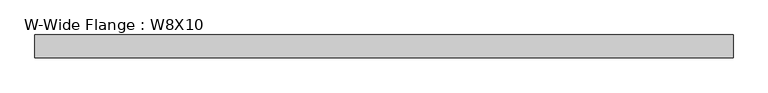
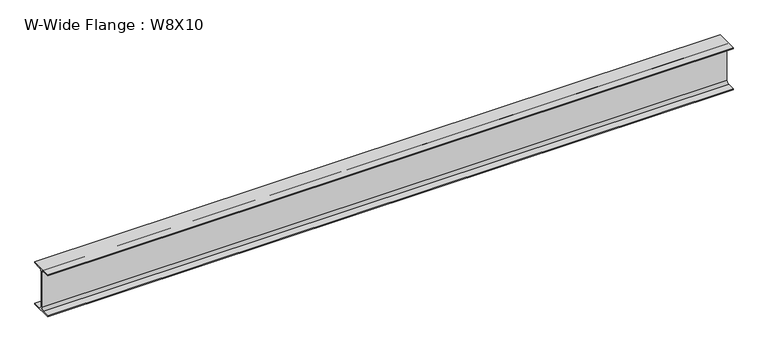
"""IFC4 building model written with IfcOpenShell, lengths in millimetres: beam geometry, W-Wide Flange : W8X10."""

from ifc_helpers import new_model, si_unit, point, frame, frame_2d, origin, place, context, project, spatial, polyline, circle_curve, trimmed, segment, composite_curve, outline, extrude, source, transform, mapped, element, save


def w_wide_flange_w8x10_f623109c(model_context):
    return source(origin(), model_context, "Body", "SweptSolid", [
        extrude(outline(composite_curve([segment(polyline([(50.038, -94.996), (50.038, -100.203), (-50.038, -100.203), (-50.038, -94.996), (-14.4145, -94.996)]), True, "CONTINUOUS"), segment(trimmed(circle_curve(frame_2d((-14.4145, -82.7405)), 12.2555), [point((-14.4145, -94.996))], [point((-2.159, -82.7405))], True, "CARTESIAN"), True, "CONTINUOUS"), segment(polyline([(-2.159, -82.7405), (-2.159, 82.7405)]), True, "CONTINUOUS"), segment(trimmed(circle_curve(frame_2d((-14.4145, 82.7405)), 12.2555), [point((-2.159, 82.7405))], [point((-14.4145, 94.996))], True, "CARTESIAN"), True, "CONTINUOUS"), segment(polyline([(-14.4145, 94.996), (-50.038, 94.996), (-50.038, 100.203), (50.038, 100.203), (50.038, 94.996), (14.4145, 94.996)]), True, "CONTINUOUS"), segment(trimmed(circle_curve(frame_2d((14.4145, 82.7405)), 12.2555), [point((14.4145, 94.996))], [point((2.159, 82.7405))], True, "CARTESIAN"), True, "CONTINUOUS"), segment(polyline([(2.159, 82.7405), (2.159, -82.7405)]), True, "CONTINUOUS"), segment(trimmed(circle_curve(frame_2d((14.4145, -82.7405)), 12.2555), [point((2.159, -82.7405))], [point((14.4145, -94.996))], True, "CARTESIAN"), True, "CONTINUOUS"), segment(polyline([(14.4145, -94.996), (50.038, -94.996)]), True, "CONTINUOUS")], self_intersect=False)), frame((-1537.4441406, 0.0, 0.0), z_axis=(1.0, 0.0, 0.0), x_axis=(0.0, 1.0, 0.0)), (0.0, 0.0, 1.0), 3074.8882813),
    ])


if __name__ == "__main__":
    model = new_model("IFC4")
    model_context = context("Model", 3, world=origin())
    ifc_project = project(units=[si_unit("LENGTHUNIT", "METRE", prefix="MILLI")], contexts=[model_context])
    site = spatial("IfcSite", under=ifc_project)
    building = spatial("IfcBuilding", under=site)
    placement = place(None, origin())
    w_wide_flange_w8x10_shape = w_wide_flange_w8x10_f623109c(model_context)
    element("IfcBeam", 1, ObjectType="W-Wide Flange : W8X10", at=placement, inside=building, context=model_context, shape_type="MappedRepresentation", body=[
        mapped(w_wide_flange_w8x10_shape, transform((0.0, 0.0, 0.0), x_axis=(1.0, 0.0, 0.0), y_axis=(0.0, 1.0, 0.0), z_axis=(0.0, 0.0, 1.0))),
    ])
    save(model, "model.ifc")

# Revit data of these elements
# Type "W-Wide Flange : W8X10"
#   Assembly Code = "B10"
#   W = 10
#   Length [instance default] = 1524 mm
#   bf = 100.076 mm
#   d = 200.406 mm
#   k = 17.463 mm
#   k2 = 12.255 mm
#   tf = 5.207 mm
#   tw = 4.318 mm
#   A = 0.00190967 m²
#   Structural Material [instance default] = Steel ASTM A992
# Element 1 (IfcBeam, "W-Wide Flange : W8X10")
#   Structural Material = Aluminum, Anodized Red
#   Materials on its faces: "Aluminum, Anodized Red"
# Materials
#   "Steel ASTM A992": class "Metal", colour RGB 128 0 0, transparency 0, Description = "Structural steel 50ksi", Cost = 0
#   "Aluminum, Anodized Red": class "Metal", colour RGB 120 120 120, transparency 0, Description = "Anodized aluminum, red", Cost = 0
